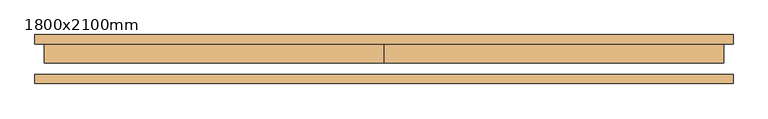
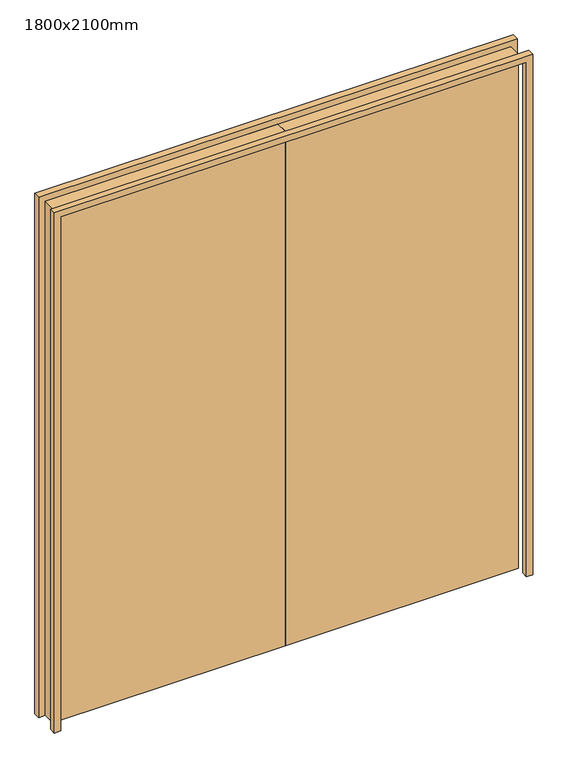
"""IFC4 building model written with IfcOpenShell, lengths in millimetres: door geometry, WWm-DoubleSolid-Flush : 1800x2100mm."""

from ifc_helpers import new_model, si_unit, frame, origin, origin_with_axes, place, context, project, spatial, polyline, outline, extrude, source, transform, mapped, element, save


def door_1800x2100mm_16297d24(model_context):
    return source(origin(), model_context, "Body", "SweptSolid", [
        extrude(outline(polyline([(0.0, 40.0), (900.0, 40.0), (900.0, -10.0), (0.0, -10.0), (0.0, 40.0)])), origin_with_axes(), (0.0, 0.0, 1.0), 2100.0),
        extrude(outline(polyline([(-900.0, 40.0), (0.0, 40.0), (0.0, -10.0), (-900.0, -10.0), (-900.0, 40.0)])), origin_with_axes(), (0.0, 0.0, 1.0), 2100.0),
        extrude(outline(polyline([(2100.0, -900.0), (2100.0, 900.0), (0.0, 900.0), (0.0, 925.0), (2125.0, 925.0), (2125.0, -925.0), (0.0, -925.0), (0.0, -900.0), (2100.0, -900.0)])), frame((0.0, -65.0, 0.0), z_axis=(0.0, 1.0, 0.0), x_axis=(0.0, 0.0, 1.0)), (0.0, 0.0, 1.0), 25.0),
        extrude(outline(polyline([(2100.0, -900.0), (2100.0, 900.0), (0.0, 900.0), (0.0, 925.0), (2125.0, 925.0), (2125.0, -925.0), (0.0, -925.0), (0.0, -900.0), (2100.0, -900.0)])), frame((0.0, 40.0, 0.0), z_axis=(0.0, 1.0, 0.0), x_axis=(0.0, 0.0, 1.0)), (0.0, 0.0, 1.0), 25.0),
    ])


if __name__ == "__main__":
    model = new_model("IFC4")
    model_context = context("Model", 3, world=origin())
    ifc_project = project(units=[si_unit("LENGTHUNIT", "METRE", prefix="MILLI")], contexts=[model_context])
    site = spatial("IfcSite", under=ifc_project)
    building = spatial("IfcBuilding", under=site)
    placement = place(None, origin())
    door_1800x2100mm_shape = door_1800x2100mm_16297d24(model_context)
    element("IfcDoor", 1, ObjectType="WWm-DoubleSolid-Flush : 1800x2100mm", at=placement, inside=building, context=model_context, shape_type="MappedRepresentation", body=[
        mapped(door_1800x2100mm_shape, transform((0.0, 0.0, 0.0), x_axis=(1.0, 0.0, 0.0), y_axis=(0.0, 1.0, 0.0), z_axis=(0.0, 0.0, 1.0))),
    ])
    save(model, "model.ifc")

# Revit data of these elements
# Type "WWm-DoubleSolid-Flush : 1800x2100mm"
#   Type Mark = "EX1-44"
#   Construction Type Id = "MDOOR"
#   Assembly Code = "C1020"
#   Analytic Construction = "Metal"
#   Thickness = 50 mm
#   Thermal Resistance (R) = 0.270117 (m²·K)/W
#   Heat Transfer Coefficient (U) = 3.7021 W/(m²·K)
#   Height = 2100 mm
#   Trim Projection Ext = 25 mm
#   Trim Projection Int = 25 mm
#   Trim Width = 25 mm
#   Width = 1800 mm
#   Not 90 Degree [instance default] = no
#   90 Degree [instance default] = yes
#   Door Material = WW-EC-RGB-White
#   Frame Material = WW-EC-RGB-White
#   Visual Light Transmittance = 0
#   Solar Heat Gain Coefficient = 0
#   Function = (empty or 0)
#   Wall Closure = (empty or 0)
# Element 1 (IfcDoor, "WWm-DoubleSolid-Flush : 1800x2100mm")
#   Materials on its faces: "WW-EC-RGB-White"
# Materials
#   "WW-EC-RGB-White": class "Generic", colour RGB 255 255 255, transparency 0, Comments = "If region requests off-white, swith asset color to RGB 231-228-220", Description = "Generic Color", Cost = 0
